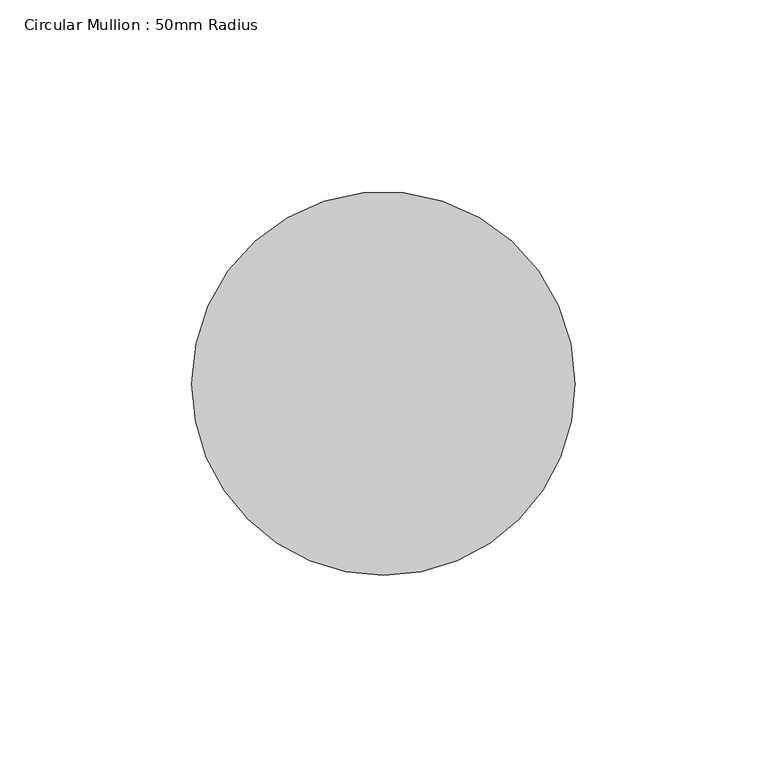
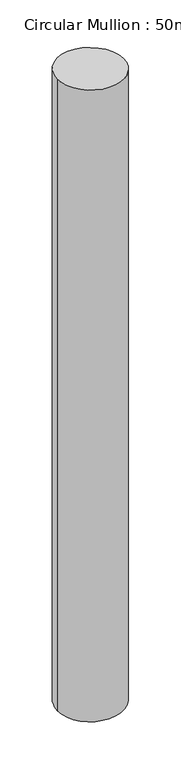
"""IFC4 building model written with IfcOpenShell, lengths in millimetres: member geometry, Circular Mullion : 50mm Radius."""

from ifc_helpers import new_model, si_unit, frame, origin, place, context, project, spatial, ellipse_curve, source, transform, mapped, element, save
from ifc_brep_helpers import plane_surface, cylinder_surface, advanced_brep


def circular_mullion_50mm_radius_4161b663(model_context):
    return source(origin(), model_context, "Body", "AdvancedBrep", [
        advanced_brep(
        [(-100.0, 0.0, 1.6734271), (0.0, 0.0, 0.0), (0.0, 0.0, -1005.6573944), (-100.0, 0.0, -1007.3423675)],
        [
            (0, 1, ellipse_curve(frame((-50.0, 0.0, 0.8367136), z_axis=(-0.01673013943324189, -0.014623606820385568, -0.9997530957982113), x_axis=(-0.7527311503281335, -0.6579529374383797, 0.02222042848129652)), 50.0123483, 50.0)),
            (1, 2),
            (2, 3, ellipse_curve(frame((-50.0, 0.0, -1006.499881), z_axis=(-0.016845513568927523, -0.014724453917580456, 0.9997496782342209), x_axis=(0.7527285771859406, 0.6579506882867877, 0.0223736646656677)), 50.0125192, 50.0)),
            (3, 0),
            (1, 0, ellipse_curve(frame((-50.0, 0.0, 0.8367136), z_axis=(-0.01673013943324189, -0.014623606820385568, -0.9997530957982113), x_axis=(-0.7527311503281335, -0.6579529374383797, 0.02222042848129652)), 50.0123483, 50.0)),
            (3, 2, ellipse_curve(frame((-50.0, 0.0, -1006.499881), z_axis=(-0.016845513568927523, -0.014724453917580456, 0.9997496782342209), x_axis=(0.7527285771859406, 0.6579506882867877, 0.0223736646656677)), 50.0125192, 50.0)),
        ],
        [
            cylinder_surface(frame((-50.0, 0.0, 0.0), z_axis=(0.0, 0.0, 1.0), x_axis=(1.0, 0.0, 0.0)), 50.0),
            plane_surface(frame((-200.5935827, 229.4891164, 0.0), z_axis=(0.01673013943324189, 0.014623606820385568, 0.9997530957982113), x_axis=(0.7527311503281338, 0.6579529374383792, -0.02222042848130842))),
            plane_surface(frame((-200.5935827, 229.4891164, -1005.6573944), z_axis=(0.016845513568927523, 0.014724453917580456, -0.9997496782342209), x_axis=(0.7527285771859407, 0.6579506882867877, 0.02237366466567048))),
        ],
        [
            (0, [[1, 2, 3, 4]]),
            (0, [[5, -4, 6, -2]]),
            (1, [[-1, -5]]),
            (2, [[-6, -3]]),
        ],
    ),
    ])


if __name__ == "__main__":
    model = new_model("IFC4")
    model_context = context("Model", 3, world=origin())
    ifc_project = project(units=[si_unit("LENGTHUNIT", "METRE", prefix="MILLI")], contexts=[model_context])
    site = spatial("IfcSite", under=ifc_project)
    building = spatial("IfcBuilding", under=site)
    placement = place(None, origin())
    circular_mullion_50mm_radius_shape = circular_mullion_50mm_radius_4161b663(model_context)
    element("IfcMember", 1, ObjectType="Circular Mullion : 50mm Radius", at=placement, inside=building, context=model_context, shape_type="MappedRepresentation", body=[
        mapped(circular_mullion_50mm_radius_shape, transform((0.0, 0.0, 0.0), x_axis=(1.0, 0.0, 0.0), y_axis=(0.0, 1.0, 0.0), z_axis=(0.0, 0.0, 1.0))),
    ])
    save(model, "model.ifc")

# Revit data of these elements
# Type "Circular Mullion : 50mm Radius"
#   built-in parameter 1007350 = 0.164042 (stored number, unit not read)
# Element 1 (IfcMember, "Circular Mullion : 50mm Radius")
#   Materials on its faces: "Aluminium"
# Materials
#   "Aluminium": class "Metal", colour RGB 247 247 247, transparency 0, Description = "Aluminium 6061", Cost = 0
